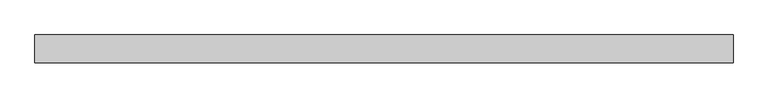
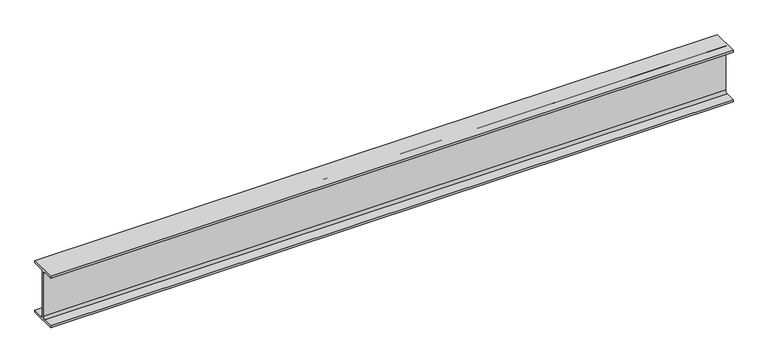
"""IFC4 building model written with IfcOpenShell, lengths in millimetres: beam geometry, 0912_Steel Framing_H-KSD3502 : H_SB_ASB_H-250x125x6x9."""

from ifc_helpers import new_model, si_unit, point, frame, frame_2d, origin, place, context, project, spatial, polyline, circle_curve, trimmed, segment, composite_curve, outline, extrude, source, transform, mapped, element, save


def beam_cd7e6579(model_context):
    return source(origin(), model_context, "Body", "SweptSolid", [
        extrude(outline(composite_curve([segment(polyline([(62.5, -116.0), (62.5, -125.0), (-62.5, -125.0), (-62.5, -116.0), (-15.0, -116.0)]), True, "CONTINUOUS"), segment(trimmed(circle_curve(frame_2d((-15.0, -104.0)), 12.0), [point((-15.0, -116.0))], [point((-3.0, -104.0))], True, "CARTESIAN"), True, "CONTINUOUS"), segment(polyline([(-3.0, -104.0), (-3.0, 104.0)]), True, "CONTINUOUS"), segment(trimmed(circle_curve(frame_2d((-15.0, 104.0)), 12.0), [point((-3.0, 104.0))], [point((-15.0, 116.0))], True, "CARTESIAN"), True, "CONTINUOUS"), segment(polyline([(-15.0, 116.0), (-62.5, 116.0), (-62.5, 125.0), (62.5, 125.0), (62.5, 116.0), (15.0, 116.0)]), True, "CONTINUOUS"), segment(trimmed(circle_curve(frame_2d((15.0, 104.0)), 12.0), [point((15.0, 116.0))], [point((3.0, 104.0))], True, "CARTESIAN"), True, "CONTINUOUS"), segment(polyline([(3.0, 104.0), (3.0, -104.0)]), True, "CONTINUOUS"), segment(trimmed(circle_curve(frame_2d((15.0, -104.0)), 12.0), [point((3.0, -104.0))], [point((15.0, -116.0))], True, "CARTESIAN"), True, "CONTINUOUS"), segment(polyline([(15.0, -116.0), (62.5, -116.0)]), True, "CONTINUOUS")], self_intersect=False)), frame((-1654.8000435, 0.0, 0.0), z_axis=(1.0, 0.0, 0.0), x_axis=(0.0, 1.0, 0.0)), (0.0, 0.0, 1.0), 3149.2888185),
    ])


if __name__ == "__main__":
    model = new_model("IFC4")
    model_context = context("Model", 3, world=origin())
    ifc_project = project(units=[si_unit("LENGTHUNIT", "METRE", prefix="MILLI")], contexts=[model_context])
    site = spatial("IfcSite", under=ifc_project)
    building = spatial("IfcBuilding", under=site)
    placement = place(None, origin())
    beam_shape = beam_cd7e6579(model_context)
    element("IfcBeam", 1, ObjectType="0912_Steel Framing_H-KSD3502 : H_SB_ASB_H-250x125x6x9", at=placement, inside=building, context=model_context, shape_type="MappedRepresentation", body=[
        mapped(beam_shape, transform((0.0, 0.0, 0.0), x_axis=(1.0, 0.0, 0.0), y_axis=(0.0, 1.0, 0.0), z_axis=(0.0, 0.0, 1.0))),
    ])
    save(model, "model.ifc")

# Revit data of these elements
# Type "0912_Steel Framing_H-KSD3502 : H_SB_ASB_H-250x125x6x9"
#   H_WM Code_1 = "S01AA003-00001 | Main Steel Structure Fabrication Work | Shelter/Building | Light Steel - Standard (30KG/M>Weight) | Material: (   )"
#   H_WM Code_2 = "S03AA029-00001 | Main Steel Structure Erection Work | Shelter/Building | Light Steel (30KG/M>Weight) | Material: (   )"
#   H_WM Code_3 = "S01AA010-00001 | Main Steel Structure Fabrication Work | Shelter/Building | Steel Painting/Coating | for Non-Fireproofed Steel Surface, Surface Preparation, Primer, Second & Final Coat | Material: (   )"
#   H_Q'ty Cal Type Tag = "SB-Q2"
#   Width = 12.5 cm
#   Web Thickness = 0.6 cm
#   Web Fillet = 1.2 cm
#   Warping Constant = 42539.8 cm⁶
#   W = 0
#   Torsional Moment of Inertia = 7.8102 cm⁴
#   Section Area = 37.66 cm²
#   Plastic Modulus weak axis = 73.1 cm³
#   Plastic Modulus strong axis = 366.0 cm³
#   Perimeter = 0.97 m²/m
#   Nominal Weight = 29.60 kgf/m
#   Moment of Inertia weak axis = 294.00 cm⁴
#   Moment of Inertia strong axis = 4050.00 cm⁴
#   Height = 25.0 cm
#   Flange Thickness = 0.9 cm
#   Elastic Modulus weak axis = 47.0 cm³
#   Elastic Modulus strong axis = 324.0 cm³
#   Centroid Vertical = 12.5 cm
#   Centroid Horizontal = 6.25 cm
#   Ix = 40500000
#   Length [instance default] = 1.5240 m
#   Zx = 366000
#   b = 0.1250 m
#   h = 0.2500 m
#   r = 0.0120 m
#   s = 0.0060 m
#   t = 0.0090 m
#   A = 0.003766 m²
#   Structural Material [instance default] = Steel, 45-345
#   Assembly Code = ""
# Element 1 (IfcBeam, "0912_Steel Framing_H-KSD3502 : H_SB_ASB_H-250x125x6x9")
#   Structural Material = none
# Materials
#   "Steel, 45-345": class "Metal", colour RGB 189 187 185, transparency 0, Description = "Steel 345 MPa", Cost = 0
